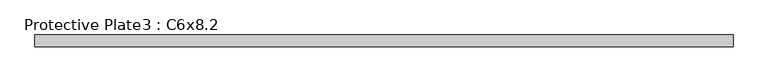
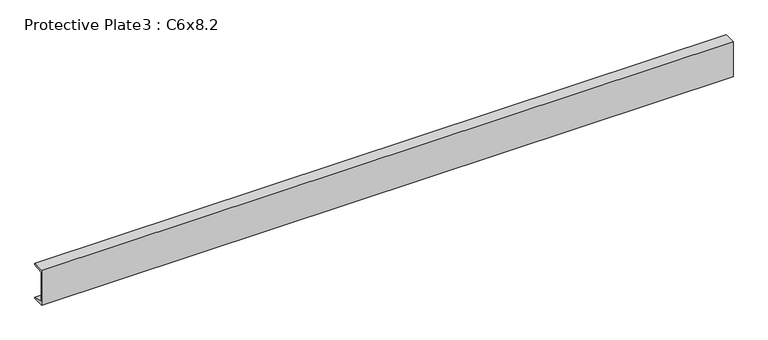
"""IFC4 building model written with IfcOpenShell, lengths in millimetres: proxy geometry, Protective Plate3 : C6x8.2."""

from ifc_helpers import new_model, si_unit, frame, origin, place, context, project, spatial, polyline, outline, extrude, source, transform, mapped, element, save


def protective_plate3_c6x8_2_5f1a67c2(model_context):
    return source(origin(), model_context, "Body", "SweptSolid", [
        extrude(outline(polyline([(-531775.7413841, 914.4), (-531775.7413841, 909.32), (-531819.4492278, 901.6131279), (-531819.4492278, 774.7868721), (-531775.7413841, 767.08), (-531775.7413841, 762.0), (-531824.5093841, 762.0), (-531824.5093841, 914.4), (-531775.7413841, 914.4)])), frame((587416.6934739, 0.0, 0.0), z_axis=(1.0, 0.0, 0.0), x_axis=(0.0, 1.0, 0.0)), (0.0, 0.0, 1.0), 2854.7900527),
    ])


if __name__ == "__main__":
    model = new_model("IFC4")
    model_context = context("Model", 3, world=origin())
    ifc_project = project(units=[si_unit("LENGTHUNIT", "METRE", prefix="MILLI")], contexts=[model_context])
    site = spatial("IfcSite", under=ifc_project)
    building = spatial("IfcBuilding", under=site)
    placement = place(None, origin())
    protective_plate3_c6x8_2_shape = protective_plate3_c6x8_2_5f1a67c2(model_context)
    element("IfcBuildingElementProxy", 1, Name="Protective Plate3 : C6x8.2", ObjectType="Protective Plate3 : C6x8.2", at=placement, inside=building, context=model_context, shape_type="MappedRepresentation", body=[
        mapped(protective_plate3_c6x8_2_shape, transform((0.0, 0.0, 0.0), x_axis=(1.0, 0.0, 0.0), y_axis=(0.0, 1.0, 0.0), z_axis=(0.0, 0.0, 1.0))),
    ])
    save(model, "model.ifc")

# Revit data of these elements
# Element 1 (IfcBuildingElementProxy, "Protective Plate3 : C6x8.2")
#   Materials on its faces: "C6x8.2 GALV CHANNEL"
# Materials
#   "C6x8.2 GALV CHANNEL": class "Generic", colour RGB 211 211 207, transparency 0, Cost = 0
